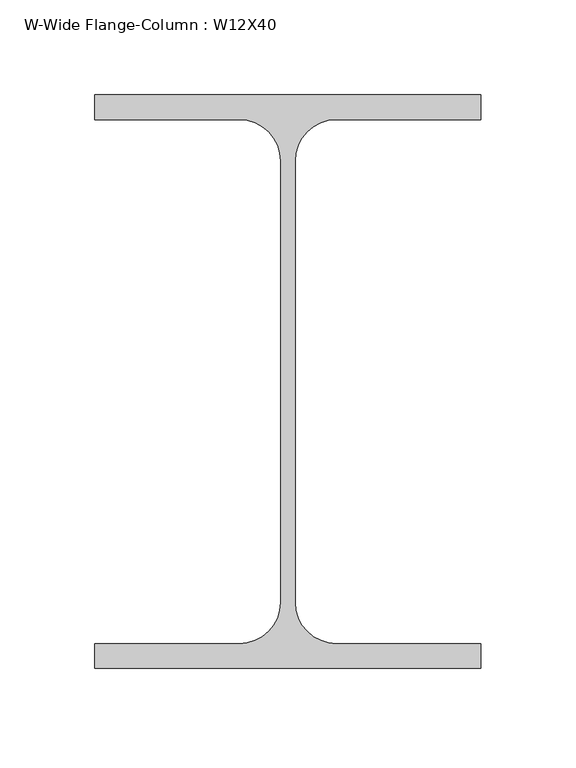
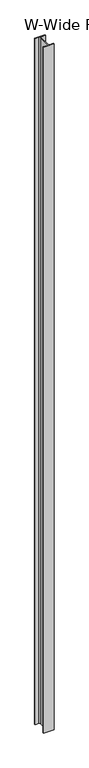
"""IFC4 building model written with IfcOpenShell, lengths in millimetres: column geometry, W-Wide Flange-Column : W12X40."""

import ifcopenshell
import ifcopenshell.guid

model = None  # the IFC model being written
_history = None  # IfcOwnerHistory: only IFC2X3 demands one
_inside = {}  # id of a spatial element -> (the spatial element, [elements in it])
_under = {}  # id of a project, library or spatial element -> (it, [spatial elements below it])
_declared = {}  # id of a project -> (the project, [libraries it declares])
_typed = {}  # id of a type object -> (the type object, [elements of that type])
_made_of = {}  # id of a material, layer set ... -> (it, [elements and type objects made of it])


def new_model(schema):
    """Start an empty IFC model of exactly this schema.

    Asked for "IFC4X3", IfcOpenShell would pick the latest addendum, in which some entities
    have other attributes; the version numbers below select the first issue.
    IFC2X3 requires an IfcOwnerHistory on every rooted entity: one is made here for all.
    """
    global model, _history
    if schema == "IFC4X3":
        model = ifcopenshell.file(schema_version=(4, 3, 0, 0))
    else:
        model = ifcopenshell.file(schema=schema)
    _inside.clear()
    _under.clear()
    _declared.clear()
    _typed.clear()
    _made_of.clear()
    _history = None
    if model.schema == "IFC2X3":
        org = make("IfcOrganization", Name="unknown")
        user = make(
            "IfcPersonAndOrganization",
            ThePerson=make("IfcPerson", FamilyName="unknown"),
            TheOrganization=org,
        )
        app = make(
            "IfcApplication",
            ApplicationDeveloper=org,
            Version="unknown",
            ApplicationFullName="unknown",
            ApplicationIdentifier="unknown",
        )
        _history = make(
            "IfcOwnerHistory",
            OwningUser=user,
            OwningApplication=app,
            ChangeAction="ADDED",
            CreationDate=0,
        )
    return model


def make(cls, **values):
    """One entity of the class cls with the attributes given. An attribute that is None is left unset."""
    return model.create_entity(
        cls, **{name: value for name, value in values.items() if value is not None}
    )


def rooted(cls, **values):
    """An entity with a GlobalId (a new one), such as an element, a storey or a relation."""
    return make(cls, GlobalId=ifcopenshell.guid.new(), OwnerHistory=_history, **values)


def si_unit(unit_type, name, prefix=None):
    """IfcSIUnit, for example si_unit("LENGTHUNIT", "METRE", prefix="MILLI")."""
    return make("IfcSIUnit", UnitType=unit_type, Prefix=prefix, Name=name)


def assignment(units):
    """IfcUnitAssignment: the units of a project."""
    return None if units is None else make("IfcUnitAssignment", Units=units)


def point(xyz):
    """IfcCartesianPoint."""
    return None if xyz is None else make("IfcCartesianPoint", Coordinates=xyz)


def direction(xyz):
    """IfcDirection."""
    return None if xyz is None else make("IfcDirection", DirectionRatios=xyz)


def frame(location, z_axis=None, x_axis=None):
    """IfcAxis2Placement3D, a coordinate frame: its origin and axes. An axis left out is left unset."""
    return make(
        "IfcAxis2Placement3D",
        Location=point(location),
        Axis=direction(z_axis),
        RefDirection=direction(x_axis),
    )


def frame_2d(location, x_axis=None):
    """IfcAxis2Placement2D, a coordinate frame in the plane: its origin and x axis."""
    return make(
        "IfcAxis2Placement2D", Location=point(location), RefDirection=direction(x_axis)
    )


def origin():
    """The frame at (0, 0, 0) with its axes left unset."""
    return frame((0.0, 0.0, 0.0))


def place(relative_to, where):
    """IfcLocalPlacement: puts the frame where relative to a parent placement (None: the world)."""
    return make(
        "IfcLocalPlacement", PlacementRelTo=relative_to, RelativePlacement=where
    )


def context(
    kind, dimensions, precision=None, world=None, true_north=None, identifier=None
):
    """IfcGeometricRepresentationContext, for example the 3D "Model" context."""
    return make(
        "IfcGeometricRepresentationContext",
        ContextIdentifier=identifier,
        ContextType=kind,
        CoordinateSpaceDimension=dimensions,
        Precision=precision,
        WorldCoordinateSystem=world,
        TrueNorth=true_north,
    )


def project(units=None, contexts=None):
    """IfcProject with its units and contexts."""
    return rooted(
        "IfcProject",
        Name="project",
        RepresentationContexts=contexts,
        UnitsInContext=assignment(units),
    )


def spatial(cls, under=None, at=None, **own):
    """A site, building, storey or space (cls), placed at a placement, below another one or the project."""
    s = rooted(cls, ObjectPlacement=at, **own)
    if under is not None:
        _under.setdefault(under.id(), (under, []))[1].append(s)
    return s


def polyline(points):
    """IfcPolyline through the points."""
    return make("IfcPolyline", Points=[point(p) for p in points])


def circle_curve(where, radius):
    """IfcCircle in the frame where."""
    return make("IfcCircle", Position=where, Radius=radius)


def trimmed(basis, trim1, trim2, sense, master):
    """IfcTrimmedCurve: the piece of a basis curve between two trims."""
    return make(
        "IfcTrimmedCurve",
        BasisCurve=basis,
        Trim1=trim1,
        Trim2=trim2,
        SenseAgreement=sense,
        MasterRepresentation=master,
    )


def segment(curve, same_sense, transition):
    """IfcCompositeCurveSegment."""
    return make(
        "IfcCompositeCurveSegment",
        Transition=transition,
        SameSense=same_sense,
        ParentCurve=curve,
    )


def composite_curve(segments, self_intersect=None):
    """IfcCompositeCurve: segments joined end to end."""
    return make("IfcCompositeCurve", Segments=segments, SelfIntersect=self_intersect)


def outline(outer, holes=None, kind="AREA"):
    """IfcArbitraryClosedProfileDef: a profile drawn as a closed curve; with holes, ...WithVoids."""
    if holes is None:
        return make("IfcArbitraryClosedProfileDef", ProfileType=kind, OuterCurve=outer)
    return make(
        "IfcArbitraryProfileDefWithVoids",
        ProfileType=kind,
        OuterCurve=outer,
        InnerCurves=holes,
    )


def extrude(swept, where, along, depth):
    """IfcExtrudedAreaSolid: the profile swept, set in the frame where, extruded along a direction by depth."""
    return make(
        "IfcExtrudedAreaSolid",
        SweptArea=swept,
        Position=where,
        ExtrudedDirection=direction(along),
        Depth=depth,
    )


def shape(context_of_items, identifier, shape_type, items):
    """IfcShapeRepresentation: the items that make up one representation, for example the "Body"."""
    return make(
        "IfcShapeRepresentation",
        ContextOfItems=context_of_items,
        RepresentationIdentifier=identifier,
        RepresentationType=shape_type,
        Items=items,
    )


def source(mapping_origin, context_of_items, identifier, shape_type, items):
    """IfcRepresentationMap: a shape defined once, which mapped items show again and again."""
    return make(
        "IfcRepresentationMap",
        MappingOrigin=mapping_origin,
        MappedRepresentation=shape(context_of_items, identifier, shape_type, items),
    )


def transform(
    local_origin,
    x_axis=None,
    y_axis=None,
    z_axis=None,
    scale=None,
    scale2=None,
    scale3=None,
    uniform=True,
):
    """IfcCartesianTransformationOperator3D, or its non-uniform kind. x_axis, y_axis, z_axis: its Axis1, 2, 3."""
    if uniform:
        return make(
            "IfcCartesianTransformationOperator3D",
            Axis1=direction(x_axis),
            Axis2=direction(y_axis),
            LocalOrigin=point(local_origin),
            Scale=scale,
            Axis3=direction(z_axis),
        )
    return make(
        "IfcCartesianTransformationOperator3DnonUniform",
        Axis1=direction(x_axis),
        Axis2=direction(y_axis),
        LocalOrigin=point(local_origin),
        Scale=scale,
        Axis3=direction(z_axis),
        Scale2=scale2,
        Scale3=scale3,
    )


def mapped(mapping_source, mapping_target):
    """IfcMappedItem: shows the shape of a source again, moved by a transform."""
    return make(
        "IfcMappedItem", MappingSource=mapping_source, MappingTarget=mapping_target
    )


def made_of(thing, what):
    """Note that an element or type object is made of a material, layer set ...; save() writes the relation."""
    if what is not None:
        _made_of.setdefault(what.id(), (what, []))[1].append(thing)
    return thing


def element(
    cls,
    number,
    at=None,
    inside=None,
    cuts=None,
    type_object=None,
    material=None,
    context=None,
    identifier="Body",
    shape_type=None,
    held_by="IfcProductDefinitionShape",
    body=None,
    shapes=None,
    **own,
):
    """One element of the class cls, such as IfcWall. Its Tag is "e" and its number.

    at: its placement. inside: the storey or other place that contains it. cuts: it is an
    opening in that element (IfcRelVoidsElement). A single representation is given by context,
    identifier, shape_type and body (its items); several are given by shapes. held_by: the class
    of the entity that holds the representations. save() writes the other relations.
    """
    e = rooted(cls, Tag="e%d" % number, ObjectPlacement=at, **own)
    if body is not None:
        shapes = [shape(context, identifier, shape_type, body)]
    if shapes is not None:
        e.Representation = make(held_by, Representations=shapes)
    if inside is not None:
        _inside.setdefault(inside.id(), (inside, []))[1].append(e)
    if cuts is not None:
        rooted(
            "IfcRelVoidsElement", RelatingBuildingElement=cuts, RelatedOpeningElement=e
        )
    if type_object is not None:
        _typed.setdefault(type_object.id(), (type_object, []))[1].append(e)
    return made_of(e, material)


def aggregate(whole, parts):
    """IfcRelAggregates: a whole, such as a stair, and the parts it consists of."""
    return rooted("IfcRelAggregates", RelatingObject=whole, RelatedObjects=parts)


def save(model, path):
    """Write the relations noted so far, then the file.

    IfcRelAggregates (storeys below a building ...), IfcRelContainedInSpatialStructure (elements
    in a storey), IfcRelDefinesByType, IfcRelAssociatesMaterial and IfcRelDeclares: one each for
    every whole, place, type object, material and project.
    """
    for whole, parts in _under.values():
        aggregate(whole, parts)
    for where, things in _inside.values():
        rooted(
            "IfcRelContainedInSpatialStructure",
            RelatedElements=things,
            RelatingStructure=where,
        )
    for kind, things in _typed.values():
        rooted("IfcRelDefinesByType", RelatedObjects=things, RelatingType=kind)
    for what, things in _made_of.values():
        rooted("IfcRelAssociatesMaterial", RelatedObjects=things, RelatingMaterial=what)
    for by, libraries in _declared.values():
        rooted("IfcRelDeclares", RelatingContext=by, RelatedDefinitions=libraries)
    model.write(path)


def w_wide_flange_column_w12x40_01d1a46c(model_context):
    return source(origin(), model_context, "Body", "SweptSolid", [
        extrude(outline(composite_curve([segment(polyline([(101.727, 151.13), (101.727, 138.049), (25.5905, 138.049)]), True, "CONTINUOUS"), segment(trimmed(circle_curve(frame_2d((25.5905, 116.205)), 21.844), [point((25.5905, 138.049))], [point((3.7465, 116.205))], True, "CARTESIAN"), True, "CONTINUOUS"), segment(polyline([(3.7465, 116.205), (3.7465, -116.205)]), True, "CONTINUOUS"), segment(trimmed(circle_curve(frame_2d((25.5905, -116.205)), 21.844), [point((3.7465, -116.205))], [point((25.5905, -138.049))], True, "CARTESIAN"), True, "CONTINUOUS"), segment(polyline([(25.5905, -138.049), (101.727, -138.049), (101.727, -151.13), (-101.727, -151.13), (-101.727, -138.049), (-25.5905, -138.049)]), True, "CONTINUOUS"), segment(trimmed(circle_curve(frame_2d((-25.5905, -116.205)), 21.844), [point((-25.5905, -138.049))], [point((-3.7465, -116.205))], True, "CARTESIAN"), True, "CONTINUOUS"), segment(polyline([(-3.7465, -116.205), (-3.7465, 116.205)]), True, "CONTINUOUS"), segment(trimmed(circle_curve(frame_2d((-25.5905, 116.205)), 21.844), [point((-3.7465, 116.205))], [point((-25.5905, 138.049))], True, "CARTESIAN"), True, "CONTINUOUS"), segment(polyline([(-25.5905, 138.049), (-101.727, 138.049), (-101.727, 151.13), (101.727, 151.13)]), True, "CONTINUOUS")], self_intersect=False)), frame((0.0, 0.0, 13379.45), z_axis=(0.0, 0.0, 1.0), x_axis=(1.0, 0.0, 0.0)), (0.0, 0.0, 1.0), 14204.95),
    ])


if __name__ == "__main__":
    model = new_model("IFC4")
    model_context = context("Model", 3, world=origin())
    ifc_project = project(units=[si_unit("LENGTHUNIT", "METRE", prefix="MILLI")], contexts=[model_context])
    site = spatial("IfcSite", under=ifc_project)
    building = spatial("IfcBuilding", under=site)
    placement = place(None, origin())
    w_wide_flange_column_w12x40_shape = w_wide_flange_column_w12x40_01d1a46c(model_context)
    element("IfcColumn", 1, ObjectType="W-Wide Flange-Column : W12X40", at=placement, inside=building, context=model_context, shape_type="MappedRepresentation", body=[
        mapped(w_wide_flange_column_w12x40_shape, transform((0.0, 0.0, 0.0), x_axis=(1.0, 0.0, 0.0), y_axis=(0.0, 1.0, 0.0), z_axis=(0.0, 0.0, 1.0))),
    ])
    save(model, "model.ifc")

# Revit data of these elements
# Type "W-Wide Flange-Column : W12X40"
#   Assembly Code = "B10"
#   W = 40
#   bf = 0' - 8.01"
#   d = 0' - 11.9"
#   k = 0' - 1 3/8"
#   kr = 0' - 0.86"
#   tf = 0' - 0.515"
#   tw = 0' - 0.295"
#   A = 0.08125 SF
#   Structural Material [instance default] = Steel ASTM A992
# Element 1 (IfcColumn, "W-Wide Flange-Column : W12X40")
#   Materials on its faces: "Steel ASTM A992"
# Materials
#   "Steel ASTM A992": class "Metal", colour RGB 199 199 199, transparency 0, Description = "Structural steel 50ksi", Cost = 0
